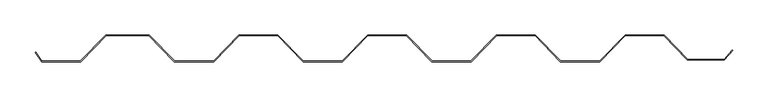
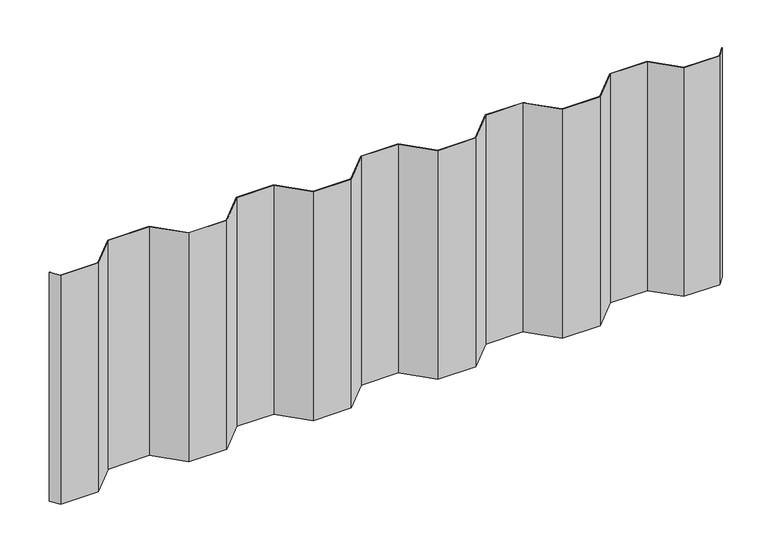
"""IFC4 building model written with IfcOpenShell, lengths in millimetres: proxy geometry, Generic Models 2:Generic Models 2:310765:Generic Models 2:310765 : Generic Models 2:Generic Models 2:310765:3 : Generic Models 2:Generic Models 2:310765:Generic Models 2:310765 : Generic Models 2:Generic Models 2:310765:300385."""

import ifcopenshell
import ifcopenshell.guid

model = None  # the IFC model being written
_history = None  # IfcOwnerHistory: only IFC2X3 demands one
_inside = {}  # id of a spatial element -> (the spatial element, [elements in it])
_under = {}  # id of a project, library or spatial element -> (it, [spatial elements below it])
_declared = {}  # id of a project -> (the project, [libraries it declares])
_typed = {}  # id of a type object -> (the type object, [elements of that type])
_made_of = {}  # id of a material, layer set ... -> (it, [elements and type objects made of it])


def new_model(schema):
    """Start an empty IFC model of exactly this schema.

    Asked for "IFC4X3", IfcOpenShell would pick the latest addendum, in which some entities
    have other attributes; the version numbers below select the first issue.
    IFC2X3 requires an IfcOwnerHistory on every rooted entity: one is made here for all.
    """
    global model, _history
    if schema == "IFC4X3":
        model = ifcopenshell.file(schema_version=(4, 3, 0, 0))
    else:
        model = ifcopenshell.file(schema=schema)
    _inside.clear()
    _under.clear()
    _declared.clear()
    _typed.clear()
    _made_of.clear()
    _history = None
    if model.schema == "IFC2X3":
        org = make("IfcOrganization", Name="unknown")
        user = make(
            "IfcPersonAndOrganization",
            ThePerson=make("IfcPerson", FamilyName="unknown"),
            TheOrganization=org,
        )
        app = make(
            "IfcApplication",
            ApplicationDeveloper=org,
            Version="unknown",
            ApplicationFullName="unknown",
            ApplicationIdentifier="unknown",
        )
        _history = make(
            "IfcOwnerHistory",
            OwningUser=user,
            OwningApplication=app,
            ChangeAction="ADDED",
            CreationDate=0,
        )
    return model


def make(cls, **values):
    """One entity of the class cls with the attributes given. An attribute that is None is left unset."""
    return model.create_entity(
        cls, **{name: value for name, value in values.items() if value is not None}
    )


def rooted(cls, **values):
    """An entity with a GlobalId (a new one), such as an element, a storey or a relation."""
    return make(cls, GlobalId=ifcopenshell.guid.new(), OwnerHistory=_history, **values)


def si_unit(unit_type, name, prefix=None):
    """IfcSIUnit, for example si_unit("LENGTHUNIT", "METRE", prefix="MILLI")."""
    return make("IfcSIUnit", UnitType=unit_type, Prefix=prefix, Name=name)


def assignment(units):
    """IfcUnitAssignment: the units of a project."""
    return None if units is None else make("IfcUnitAssignment", Units=units)


def point(xyz):
    """IfcCartesianPoint."""
    return None if xyz is None else make("IfcCartesianPoint", Coordinates=xyz)


def direction(xyz):
    """IfcDirection."""
    return None if xyz is None else make("IfcDirection", DirectionRatios=xyz)


def frame(location, z_axis=None, x_axis=None):
    """IfcAxis2Placement3D, a coordinate frame: its origin and axes. An axis left out is left unset."""
    return make(
        "IfcAxis2Placement3D",
        Location=point(location),
        Axis=direction(z_axis),
        RefDirection=direction(x_axis),
    )


def origin():
    """The frame at (0, 0, 0) with its axes left unset."""
    return frame((0.0, 0.0, 0.0))


def place(relative_to, where):
    """IfcLocalPlacement: puts the frame where relative to a parent placement (None: the world)."""
    return make(
        "IfcLocalPlacement", PlacementRelTo=relative_to, RelativePlacement=where
    )


def context(
    kind, dimensions, precision=None, world=None, true_north=None, identifier=None
):
    """IfcGeometricRepresentationContext, for example the 3D "Model" context."""
    return make(
        "IfcGeometricRepresentationContext",
        ContextIdentifier=identifier,
        ContextType=kind,
        CoordinateSpaceDimension=dimensions,
        Precision=precision,
        WorldCoordinateSystem=world,
        TrueNorth=true_north,
    )


def project(units=None, contexts=None):
    """IfcProject with its units and contexts."""
    return rooted(
        "IfcProject",
        Name="project",
        RepresentationContexts=contexts,
        UnitsInContext=assignment(units),
    )


def spatial(cls, under=None, at=None, **own):
    """A site, building, storey or space (cls), placed at a placement, below another one or the project."""
    s = rooted(cls, ObjectPlacement=at, **own)
    if under is not None:
        _under.setdefault(under.id(), (under, []))[1].append(s)
    return s


def polyline(points):
    """IfcPolyline through the points."""
    return make("IfcPolyline", Points=[point(p) for p in points])


def outline(outer, holes=None, kind="AREA"):
    """IfcArbitraryClosedProfileDef: a profile drawn as a closed curve; with holes, ...WithVoids."""
    if holes is None:
        return make("IfcArbitraryClosedProfileDef", ProfileType=kind, OuterCurve=outer)
    return make(
        "IfcArbitraryProfileDefWithVoids",
        ProfileType=kind,
        OuterCurve=outer,
        InnerCurves=holes,
    )


def extrude(swept, where, along, depth):
    """IfcExtrudedAreaSolid: the profile swept, set in the frame where, extruded along a direction by depth."""
    return make(
        "IfcExtrudedAreaSolid",
        SweptArea=swept,
        Position=where,
        ExtrudedDirection=direction(along),
        Depth=depth,
    )


def shape(context_of_items, identifier, shape_type, items):
    """IfcShapeRepresentation: the items that make up one representation, for example the "Body"."""
    return make(
        "IfcShapeRepresentation",
        ContextOfItems=context_of_items,
        RepresentationIdentifier=identifier,
        RepresentationType=shape_type,
        Items=items,
    )


def source(mapping_origin, context_of_items, identifier, shape_type, items):
    """IfcRepresentationMap: a shape defined once, which mapped items show again and again."""
    return make(
        "IfcRepresentationMap",
        MappingOrigin=mapping_origin,
        MappedRepresentation=shape(context_of_items, identifier, shape_type, items),
    )


def transform(
    local_origin,
    x_axis=None,
    y_axis=None,
    z_axis=None,
    scale=None,
    scale2=None,
    scale3=None,
    uniform=True,
):
    """IfcCartesianTransformationOperator3D, or its non-uniform kind. x_axis, y_axis, z_axis: its Axis1, 2, 3."""
    if uniform:
        return make(
            "IfcCartesianTransformationOperator3D",
            Axis1=direction(x_axis),
            Axis2=direction(y_axis),
            LocalOrigin=point(local_origin),
            Scale=scale,
            Axis3=direction(z_axis),
        )
    return make(
        "IfcCartesianTransformationOperator3DnonUniform",
        Axis1=direction(x_axis),
        Axis2=direction(y_axis),
        LocalOrigin=point(local_origin),
        Scale=scale,
        Axis3=direction(z_axis),
        Scale2=scale2,
        Scale3=scale3,
    )


def mapped(mapping_source, mapping_target):
    """IfcMappedItem: shows the shape of a source again, moved by a transform."""
    return make(
        "IfcMappedItem", MappingSource=mapping_source, MappingTarget=mapping_target
    )


def made_of(thing, what):
    """Note that an element or type object is made of a material, layer set ...; save() writes the relation."""
    if what is not None:
        _made_of.setdefault(what.id(), (what, []))[1].append(thing)
    return thing


def element(
    cls,
    number,
    at=None,
    inside=None,
    cuts=None,
    type_object=None,
    material=None,
    context=None,
    identifier="Body",
    shape_type=None,
    held_by="IfcProductDefinitionShape",
    body=None,
    shapes=None,
    **own,
):
    """One element of the class cls, such as IfcWall. Its Tag is "e" and its number.

    at: its placement. inside: the storey or other place that contains it. cuts: it is an
    opening in that element (IfcRelVoidsElement). A single representation is given by context,
    identifier, shape_type and body (its items); several are given by shapes. held_by: the class
    of the entity that holds the representations. save() writes the other relations.
    """
    e = rooted(cls, Tag="e%d" % number, ObjectPlacement=at, **own)
    if body is not None:
        shapes = [shape(context, identifier, shape_type, body)]
    if shapes is not None:
        e.Representation = make(held_by, Representations=shapes)
    if inside is not None:
        _inside.setdefault(inside.id(), (inside, []))[1].append(e)
    if cuts is not None:
        rooted(
            "IfcRelVoidsElement", RelatingBuildingElement=cuts, RelatedOpeningElement=e
        )
    if type_object is not None:
        _typed.setdefault(type_object.id(), (type_object, []))[1].append(e)
    return made_of(e, material)


def aggregate(whole, parts):
    """IfcRelAggregates: a whole, such as a stair, and the parts it consists of."""
    return rooted("IfcRelAggregates", RelatingObject=whole, RelatedObjects=parts)


def save(model, path):
    """Write the relations noted so far, then the file.

    IfcRelAggregates (storeys below a building ...), IfcRelContainedInSpatialStructure (elements
    in a storey), IfcRelDefinesByType, IfcRelAssociatesMaterial and IfcRelDeclares: one each for
    every whole, place, type object, material and project.
    """
    for whole, parts in _under.values():
        aggregate(whole, parts)
    for where, things in _inside.values():
        rooted(
            "IfcRelContainedInSpatialStructure",
            RelatedElements=things,
            RelatingStructure=where,
        )
    for kind, things in _typed.values():
        rooted("IfcRelDefinesByType", RelatedObjects=things, RelatingType=kind)
    for what, things in _made_of.values():
        rooted("IfcRelAssociatesMaterial", RelatedObjects=things, RelatingMaterial=what)
    for by, libraries in _declared.values():
        rooted("IfcRelDeclares", RelatingContext=by, RelatedDefinitions=libraries)
    model.write(path)


def generic_models_ab14fb1e(model_context):
    return source(origin(), model_context, "Body", "SweptSolid", [
        extrude(outline(polyline([(593719.8809779, -568266.4432213), (593667.2871722, -568266.4432213), (593633.6551875, -568231.8851341), (593579.1467875, -568231.8851341), (593542.9845958, -568269.1913841), (593486.9373791, -568269.1913841), (593450.7751875, -568231.8851341), (593396.2667875, -568231.8851341), (593360.1045958, -568269.1913841), (593304.0573791, -568269.1913841), (593267.8951875, -568231.8851341), (593213.3867875, -568231.8851341), (593177.2245958, -568269.1913841), (593121.1773791, -568269.1913841), (593085.0151875, -568231.8851341), (593030.5067875, -568231.8851341), (592994.3445958, -568269.1913841), (592938.2973791, -568269.1913841), (592902.1351875, -568231.8851341), (592841.2767875, -568231.8851341), (592805.1145958, -568269.1913841), (592749.8367875, -568269.1913841), (592740.6584173, -568256.0833131), (592741.3086193, -568255.6280368), (592750.2499875, -568268.3976341), (592804.7785503, -568268.3976341), (592840.9407419, -568231.0913841), (592902.471233, -568231.0913841), (592938.6334246, -568268.3976341), (592994.0085503, -568268.3976341), (593030.1707419, -568231.0913841), (593085.351233, -568231.0913841), (593121.5134246, -568268.3976341), (593176.8885503, -568268.3976341), (593213.0507419, -568231.0913841), (593268.231233, -568231.0913841), (593304.3934246, -568268.3976341), (593359.7685503, -568268.3976341), (593395.9307419, -568231.0913841), (593451.111233, -568231.0913841), (593487.2734246, -568268.3976341), (593542.6485503, -568268.3976341), (593578.8107419, -568231.0913841), (593633.9903018, -568231.0913841), (593667.6222866, -568265.6494713), (593719.5286406, -568265.6494713), (593731.1747524, -568252.7731785), (593731.7367242, -568253.3351503), (593719.8809779, -568266.4432213)])), frame((0.0, 0.0, 4490.8395931), z_axis=(0.0, 0.0, 1.0), x_axis=(1.0, 0.0, 0.0)), (0.0, 0.0, 1.0), 355.5590195),
    ])


if __name__ == "__main__":
    model = new_model("IFC4")
    model_context = context("Model", 3, world=origin())
    ifc_project = project(units=[si_unit("LENGTHUNIT", "METRE", prefix="MILLI")], contexts=[model_context])
    site = spatial("IfcSite", under=ifc_project)
    building = spatial("IfcBuilding", under=site)
    placement = place(None, origin())
    generic_models_shape = generic_models_ab14fb1e(model_context)
    element("IfcBuildingElementProxy", 1, Name="Generic Models 2:Generic Models 2:310765:Generic Models 2:310765 : Generic Models 2:Generic Models 2:310765:3 : Generic Models 2:Generic Models 2:310765:Generic Models 2:310765 : Generic Models 2:Generic Models 2:310765:300385", ObjectType="Generic Models 2:Generic Models 2:310765:Generic Models 2:310765 : Generic Models 2:Generic Models 2:310765:3 : Generic Models 2:Generic Models 2:310765:Generic Models 2:310765 : Generic Models 2:Generic Models 2:310765:300385", at=placement, inside=building, context=model_context, shape_type="MappedRepresentation", body=[
        mapped(generic_models_shape, transform((0.0, 0.0, 0.0), x_axis=(1.0, 0.0, 0.0), y_axis=(0.0, 1.0, 0.0), z_axis=(0.0, 0.0, 1.0))),
    ])
    save(model, "model.ifc")

# Revit data of these elements
# Type "Generic Models 2:Generic Models 2:310765:Generic Models 2:310765 : Generic Models 2:Generic Models 2:310765:3 : Generic Models 2:Generic Models 2:310765:Generic Models 2:310765 : Generic Models 2:Generic Models 2:310765:300385"
#   NameOverride = "Generic Models 2:Generic Models 2:310765:Generic Models 2:310765 : Generic Models 2:Generic Models 2:310765:300385"
#   ObjectTypeOverride = "Generic Models 2:310765 : Generic Models 2:Generic Models 2:310765"
#   Reference = "Generic Models 2"
#   Tag = "300385"
# Element 1 (IfcBuildingElementProxy, "Generic Models 2:Generic Models 2:310765:Generic Models 2:310765 : Generic Models 2:Generic Models 2:310765:3 : Generic Models 2:Generic Models 2:310765:Generic Models 2:310765 : Generic Models 2:Generic Models 2:310765:300385")
#   Materials on its faces: "VERTICAL CORRUGATED METAL PANEL - EXPOSED FASTENERS - (MBCI 7.2 PANEL)"
# Materials
#   "VERTICAL CORRUGATED METAL PANEL - EXPOSED FASTENERS - (MBCI 7.2 PANEL)": class "Generic", colour RGB 120 120 120, transparency 0, Cost = 0
